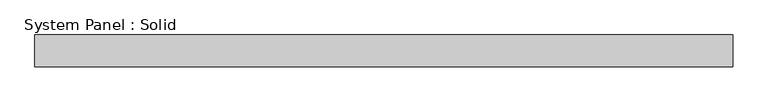
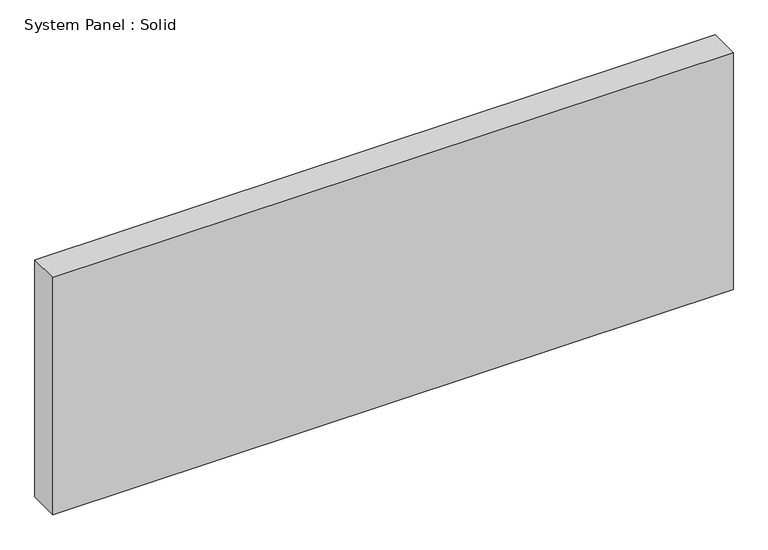
"""IFC4 building model written with IfcOpenShell, lengths in millimetres: plate geometry, System Panel : Solid."""

import ifcopenshell
import ifcopenshell.guid

model = None  # the IFC model being written
_history = None  # IfcOwnerHistory: only IFC2X3 demands one
_inside = {}  # id of a spatial element -> (the spatial element, [elements in it])
_under = {}  # id of a project, library or spatial element -> (it, [spatial elements below it])
_declared = {}  # id of a project -> (the project, [libraries it declares])
_typed = {}  # id of a type object -> (the type object, [elements of that type])
_made_of = {}  # id of a material, layer set ... -> (it, [elements and type objects made of it])


def new_model(schema):
    """Start an empty IFC model of exactly this schema.

    Asked for "IFC4X3", IfcOpenShell would pick the latest addendum, in which some entities
    have other attributes; the version numbers below select the first issue.
    IFC2X3 requires an IfcOwnerHistory on every rooted entity: one is made here for all.
    """
    global model, _history
    if schema == "IFC4X3":
        model = ifcopenshell.file(schema_version=(4, 3, 0, 0))
    else:
        model = ifcopenshell.file(schema=schema)
    _inside.clear()
    _under.clear()
    _declared.clear()
    _typed.clear()
    _made_of.clear()
    _history = None
    if model.schema == "IFC2X3":
        org = make("IfcOrganization", Name="unknown")
        user = make(
            "IfcPersonAndOrganization",
            ThePerson=make("IfcPerson", FamilyName="unknown"),
            TheOrganization=org,
        )
        app = make(
            "IfcApplication",
            ApplicationDeveloper=org,
            Version="unknown",
            ApplicationFullName="unknown",
            ApplicationIdentifier="unknown",
        )
        _history = make(
            "IfcOwnerHistory",
            OwningUser=user,
            OwningApplication=app,
            ChangeAction="ADDED",
            CreationDate=0,
        )
    return model


def make(cls, **values):
    """One entity of the class cls with the attributes given. An attribute that is None is left unset."""
    return model.create_entity(
        cls, **{name: value for name, value in values.items() if value is not None}
    )


def rooted(cls, **values):
    """An entity with a GlobalId (a new one), such as an element, a storey or a relation."""
    return make(cls, GlobalId=ifcopenshell.guid.new(), OwnerHistory=_history, **values)


def si_unit(unit_type, name, prefix=None):
    """IfcSIUnit, for example si_unit("LENGTHUNIT", "METRE", prefix="MILLI")."""
    return make("IfcSIUnit", UnitType=unit_type, Prefix=prefix, Name=name)


def assignment(units):
    """IfcUnitAssignment: the units of a project."""
    return None if units is None else make("IfcUnitAssignment", Units=units)


def point(xyz):
    """IfcCartesianPoint."""
    return None if xyz is None else make("IfcCartesianPoint", Coordinates=xyz)


def direction(xyz):
    """IfcDirection."""
    return None if xyz is None else make("IfcDirection", DirectionRatios=xyz)


def frame(location, z_axis=None, x_axis=None):
    """IfcAxis2Placement3D, a coordinate frame: its origin and axes. An axis left out is left unset."""
    return make(
        "IfcAxis2Placement3D",
        Location=point(location),
        Axis=direction(z_axis),
        RefDirection=direction(x_axis),
    )


def origin():
    """The frame at (0, 0, 0) with its axes left unset."""
    return frame((0.0, 0.0, 0.0))


def origin_with_axes():
    """The frame at (0, 0, 0) with the z axis (0, 0, 1) and the x axis (1, 0, 0) written out."""
    return frame((0.0, 0.0, 0.0), z_axis=(0.0, 0.0, 1.0), x_axis=(1.0, 0.0, 0.0))


def place(relative_to, where):
    """IfcLocalPlacement: puts the frame where relative to a parent placement (None: the world)."""
    return make(
        "IfcLocalPlacement", PlacementRelTo=relative_to, RelativePlacement=where
    )


def context(
    kind, dimensions, precision=None, world=None, true_north=None, identifier=None
):
    """IfcGeometricRepresentationContext, for example the 3D "Model" context."""
    return make(
        "IfcGeometricRepresentationContext",
        ContextIdentifier=identifier,
        ContextType=kind,
        CoordinateSpaceDimension=dimensions,
        Precision=precision,
        WorldCoordinateSystem=world,
        TrueNorth=true_north,
    )


def project(units=None, contexts=None):
    """IfcProject with its units and contexts."""
    return rooted(
        "IfcProject",
        Name="project",
        RepresentationContexts=contexts,
        UnitsInContext=assignment(units),
    )


def spatial(cls, under=None, at=None, **own):
    """A site, building, storey or space (cls), placed at a placement, below another one or the project."""
    s = rooted(cls, ObjectPlacement=at, **own)
    if under is not None:
        _under.setdefault(under.id(), (under, []))[1].append(s)
    return s


def polyline(points):
    """IfcPolyline through the points."""
    return make("IfcPolyline", Points=[point(p) for p in points])


def outline(outer, holes=None, kind="AREA"):
    """IfcArbitraryClosedProfileDef: a profile drawn as a closed curve; with holes, ...WithVoids."""
    if holes is None:
        return make("IfcArbitraryClosedProfileDef", ProfileType=kind, OuterCurve=outer)
    return make(
        "IfcArbitraryProfileDefWithVoids",
        ProfileType=kind,
        OuterCurve=outer,
        InnerCurves=holes,
    )


def extrude(swept, where, along, depth):
    """IfcExtrudedAreaSolid: the profile swept, set in the frame where, extruded along a direction by depth."""
    return make(
        "IfcExtrudedAreaSolid",
        SweptArea=swept,
        Position=where,
        ExtrudedDirection=direction(along),
        Depth=depth,
    )


def shape(context_of_items, identifier, shape_type, items):
    """IfcShapeRepresentation: the items that make up one representation, for example the "Body"."""
    return make(
        "IfcShapeRepresentation",
        ContextOfItems=context_of_items,
        RepresentationIdentifier=identifier,
        RepresentationType=shape_type,
        Items=items,
    )


def source(mapping_origin, context_of_items, identifier, shape_type, items):
    """IfcRepresentationMap: a shape defined once, which mapped items show again and again."""
    return make(
        "IfcRepresentationMap",
        MappingOrigin=mapping_origin,
        MappedRepresentation=shape(context_of_items, identifier, shape_type, items),
    )


def transform(
    local_origin,
    x_axis=None,
    y_axis=None,
    z_axis=None,
    scale=None,
    scale2=None,
    scale3=None,
    uniform=True,
):
    """IfcCartesianTransformationOperator3D, or its non-uniform kind. x_axis, y_axis, z_axis: its Axis1, 2, 3."""
    if uniform:
        return make(
            "IfcCartesianTransformationOperator3D",
            Axis1=direction(x_axis),
            Axis2=direction(y_axis),
            LocalOrigin=point(local_origin),
            Scale=scale,
            Axis3=direction(z_axis),
        )
    return make(
        "IfcCartesianTransformationOperator3DnonUniform",
        Axis1=direction(x_axis),
        Axis2=direction(y_axis),
        LocalOrigin=point(local_origin),
        Scale=scale,
        Axis3=direction(z_axis),
        Scale2=scale2,
        Scale3=scale3,
    )


def mapped(mapping_source, mapping_target):
    """IfcMappedItem: shows the shape of a source again, moved by a transform."""
    return make(
        "IfcMappedItem", MappingSource=mapping_source, MappingTarget=mapping_target
    )


def made_of(thing, what):
    """Note that an element or type object is made of a material, layer set ...; save() writes the relation."""
    if what is not None:
        _made_of.setdefault(what.id(), (what, []))[1].append(thing)
    return thing


def element(
    cls,
    number,
    at=None,
    inside=None,
    cuts=None,
    type_object=None,
    material=None,
    context=None,
    identifier="Body",
    shape_type=None,
    held_by="IfcProductDefinitionShape",
    body=None,
    shapes=None,
    **own,
):
    """One element of the class cls, such as IfcWall. Its Tag is "e" and its number.

    at: its placement. inside: the storey or other place that contains it. cuts: it is an
    opening in that element (IfcRelVoidsElement). A single representation is given by context,
    identifier, shape_type and body (its items); several are given by shapes. held_by: the class
    of the entity that holds the representations. save() writes the other relations.
    """
    e = rooted(cls, Tag="e%d" % number, ObjectPlacement=at, **own)
    if body is not None:
        shapes = [shape(context, identifier, shape_type, body)]
    if shapes is not None:
        e.Representation = make(held_by, Representations=shapes)
    if inside is not None:
        _inside.setdefault(inside.id(), (inside, []))[1].append(e)
    if cuts is not None:
        rooted(
            "IfcRelVoidsElement", RelatingBuildingElement=cuts, RelatedOpeningElement=e
        )
    if type_object is not None:
        _typed.setdefault(type_object.id(), (type_object, []))[1].append(e)
    return made_of(e, material)


def aggregate(whole, parts):
    """IfcRelAggregates: a whole, such as a stair, and the parts it consists of."""
    return rooted("IfcRelAggregates", RelatingObject=whole, RelatedObjects=parts)


def save(model, path):
    """Write the relations noted so far, then the file.

    IfcRelAggregates (storeys below a building ...), IfcRelContainedInSpatialStructure (elements
    in a storey), IfcRelDefinesByType, IfcRelAssociatesMaterial and IfcRelDeclares: one each for
    every whole, place, type object, material and project.
    """
    for whole, parts in _under.values():
        aggregate(whole, parts)
    for where, things in _inside.values():
        rooted(
            "IfcRelContainedInSpatialStructure",
            RelatedElements=things,
            RelatingStructure=where,
        )
    for kind, things in _typed.values():
        rooted("IfcRelDefinesByType", RelatedObjects=things, RelatingType=kind)
    for what, things in _made_of.values():
        rooted("IfcRelAssociatesMaterial", RelatedObjects=things, RelatingMaterial=what)
    for by, libraries in _declared.values():
        rooted("IfcRelDeclares", RelatingContext=by, RelatedDefinitions=libraries)
    model.write(path)


def system_panel_solid_037144dd(model_context):
    return source(origin(), model_context, "Body", "SweptSolid", [
        extrude(outline(polyline([(697.4416668, -44.45), (-697.4416668, -44.45), (-697.4416668, 19.05), (697.4416668, 19.05), (697.4416668, -44.45)])), origin_with_axes(), (0.0, 0.0, 1.0), 514.35),
    ])


if __name__ == "__main__":
    model = new_model("IFC4")
    model_context = context("Model", 3, world=origin())
    ifc_project = project(units=[si_unit("LENGTHUNIT", "METRE", prefix="MILLI")], contexts=[model_context])
    site = spatial("IfcSite", under=ifc_project)
    building = spatial("IfcBuilding", under=site)
    placement = place(None, origin())
    system_panel_solid_shape = system_panel_solid_037144dd(model_context)
    element("IfcPlate", 1, ObjectType="System Panel : Solid", at=placement, inside=building, context=model_context, shape_type="MappedRepresentation", body=[
        mapped(system_panel_solid_shape, transform((0.0, 0.0, 0.0), x_axis=(1.0, 0.0, 0.0), y_axis=(0.0, 1.0, 0.0), z_axis=(0.0, 0.0, 1.0))),
    ])
    save(model, "model.ifc")

# Revit data of these elements
# Project information
#   Organization Name = "G3B Press"
#   Organization Description = "Paul F. Aubin Cosulting Services, Inc."
#   Building Name = "Revit Essentials for Architecture"
#   Author = "Paul F. Aubin"
#   Author Website = "https://www.paulaubin.com"
#   Copyright = "Copyright © 2020 Paul F Aubin, all rights reserved"
#   Design Option = "Main Model"
#   Project Issue Date = "8/1/2020"
#   Project Status = "Design Development"
#   Client Name = "Working with Schedules, Tags and Data"
#   Project Address = "123 State ST\nSuite 301\nChicago, IL 60606"
#   Project Name = "13 Commercial_Complete"
#   Project Number = "2020.04A"
# Type "System Panel : Solid"
#   Construction Type Id = "MDOOR"
#   Analytic Construction = "Metal"
#   Visual Light Transmittance = 0
#   Solar Heat Gain Coefficient = 0
#   Heat Transfer Coefficient (U) = 0.651978 BTU/(h·ft²·°F)
#   Define Thermal Properties by = 1
# Element 1 (IfcPlate, "System Panel : Solid")
#   Materials on its faces: "Default"
# Materials
#   "Default": class "Miscellaneous", colour RGB 127 127 127, transparency 0, Cost = 0
